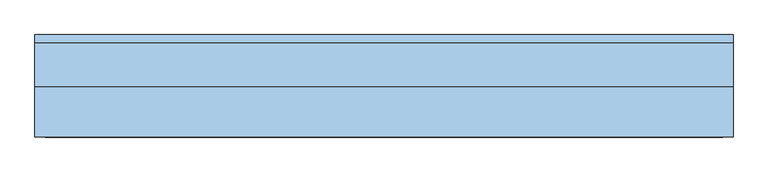
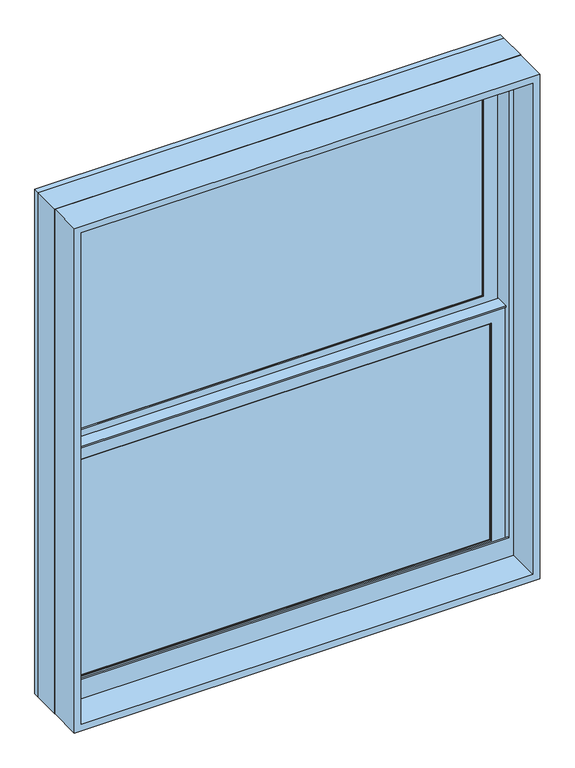
"""IFC4 building model written with IfcOpenShell, lengths in millimetres: window geometry, Window-Double_Hung-Marvin-Essential : ESDH3640."""

from ifc_helpers import new_model, si_unit, frame, origin, place, context, project, spatial, polyline, outline, extrude, faceted_brep, source, transform, mapped, element, save


def window_21e27111(model_context):
    return source(origin(), model_context, "Body", "SolidModel", [
        extrude(outline(polyline([(166.1583333, 20.6375), (166.1583333, 15.875), (147.1083333, 15.875), (147.1083333, 20.6375), (166.1583333, 20.6375)])), frame((0.0, 0.0, 1289.05), z_axis=(0.0, 0.0, 1.0), x_axis=(1.0, 0.0, 0.0)), (0.0, 0.0, 1.0), 527.05),
        extrude(outline(polyline([(-147.1083333, 20.6375), (-147.1083333, 15.875), (-166.1583333, 15.875), (-166.1583333, 20.6375), (-147.1083333, 20.6375)])), frame((0.0, 0.0, 1289.05), z_axis=(0.0, 0.0, 1.0), x_axis=(1.0, 0.0, 0.0)), (0.0, 0.0, 1.0), 527.05),
        extrude(outline(polyline([(469.9, 20.6375), (469.9, 15.875), (-469.9, 15.875), (-469.9, 20.6375), (469.9, 20.6375)])), frame((0.0, 0.0, 1543.05), z_axis=(0.0, 0.0, 1.0), x_axis=(1.0, 0.0, 0.0)), (0.0, 0.0, 1.0), 19.05),
        extrude(outline(polyline([(-166.1583333, 46.83125), (-166.1583333, 51.59375), (-147.1083333, 51.59375), (-147.1083333, 46.83125), (-166.1583333, 46.83125)])), frame((0.0, 0.0, 1854.2), z_axis=(0.0, 0.0, 1.0), x_axis=(1.0, 0.0, 0.0)), (0.0, 0.0, 1.0), 527.05),
        extrude(outline(polyline([(147.1083333, 46.83125), (147.1083333, 51.59375), (166.1583333, 51.59375), (166.1583333, 46.83125), (147.1083333, 46.83125)])), frame((0.0, 0.0, 1854.2), z_axis=(0.0, 0.0, 1.0), x_axis=(1.0, 0.0, 0.0)), (0.0, 0.0, 1.0), 527.05),
        extrude(outline(polyline([(-469.9, 46.83125), (-469.9, 51.59375), (469.9, 51.59375), (469.9, 46.83125), (-469.9, 46.83125)])), frame((0.0, 0.0, 2108.2), z_axis=(0.0, 0.0, 1.0), x_axis=(1.0, 0.0, 0.0)), (0.0, 0.0, 1.0), 19.05),
        extrude(outline(polyline([(166.1583333, 20.6375), (147.1083333, 20.6375), (147.1083333, 25.4), (166.1583333, 25.4), (166.1583333, 20.6375)])), frame((0.0, 0.0, 1289.05), z_axis=(0.0, 0.0, 1.0), x_axis=(1.0, 0.0, 0.0)), (0.0, 0.0, 1.0), 527.05),
        extrude(outline(polyline([(-147.1083333, 20.6375), (-166.1583333, 20.6375), (-166.1583333, 25.4), (-147.1083333, 25.4), (-147.1083333, 20.6375)])), frame((0.0, 0.0, 1289.05), z_axis=(0.0, 0.0, 1.0), x_axis=(1.0, 0.0, 0.0)), (0.0, 0.0, 1.0), 527.05),
        extrude(outline(polyline([(469.9, 20.6375), (-469.9, 20.6375), (-469.9, 25.4), (469.9, 25.4), (469.9, 20.6375)])), frame((0.0, 0.0, 1543.05), z_axis=(0.0, 0.0, 1.0), x_axis=(1.0, 0.0, 0.0)), (0.0, 0.0, 1.0), 19.05),
        extrude(outline(polyline([(-166.1583333, 56.35625), (-147.1083333, 56.35625), (-147.1083333, 51.59375), (-166.1583333, 51.59375), (-166.1583333, 56.35625)])), frame((0.0, 0.0, 1854.2), z_axis=(0.0, 0.0, 1.0), x_axis=(1.0, 0.0, 0.0)), (0.0, 0.0, 1.0), 527.05),
        extrude(outline(polyline([(147.1083333, 56.35625), (166.1583333, 56.35625), (166.1583333, 51.59375), (147.1083333, 51.59375), (147.1083333, 56.35625)])), frame((0.0, 0.0, 1854.2), z_axis=(0.0, 0.0, 1.0), x_axis=(1.0, 0.0, 0.0)), (0.0, 0.0, 1.0), 527.05),
        extrude(outline(polyline([(-469.9, 56.35625), (469.9, 56.35625), (469.9, 51.59375), (-469.9, 51.59375), (-469.9, 56.35625)])), frame((0.0, 0.0, 2108.2), z_axis=(0.0, 0.0, 1.0), x_axis=(1.0, 0.0, 0.0)), (0.0, 0.0, 1.0), 19.05),
        faceted_brep([(-496.8875, 5.6780605, 1846.1351748), (-496.8875, 5.6780605, 1841.5), (496.8875, 5.6780605, 1841.5), (496.8875, 5.6780605, 1846.1351748), (-496.8875, 34.8118605, 1846.1351748), (496.8875, 34.8118605, 1846.1351748), (496.8875, 34.8118605, 1841.5), (-496.8875, 34.8118605, 1841.5), (-496.8875, 30.1625, 1841.5), (-496.8875, 30.1625, 1262.0625), (-496.8875, 8.9241104, 1262.0625), (-496.8875, 8.9241104, 1841.5), (496.8875, 8.9241104, 1841.5), (496.8875, 30.1625, 1841.5), (496.8875, 8.9241104, 1262.0625), (496.8875, 30.1625, 1262.0625), (-481.0034752, 11.90625, 1827.2034752), (-481.0034752, 30.1625, 1827.2034752), (481.0034752, 30.1625, 1827.2034752), (481.0034752, 11.90625, 1827.2034752), (-464.34375, 10.4662439, 1810.54375), (-464.34375, 11.90625, 1810.54375), (464.34375, 11.90625, 1810.54375), (464.34375, 10.4662439, 1810.54375), (465.8858834, 8.9241104, 1812.0858834), (-465.8858834, 8.9241104, 1812.0858834), (481.0034752, 30.1625, 1277.9465248), (481.0034752, 11.90625, 1277.9465248), (464.34375, 11.90625, 1294.60625), (464.34375, 10.4662439, 1294.60625), (465.8858834, 8.9241104, 1293.0641166), (-481.0034752, 30.1625, 1277.9465248), (-481.0034752, 11.90625, 1277.9465248), (-464.34375, 11.90625, 1294.60625), (-464.34375, 10.4662439, 1294.60625), (-465.8858834, 8.9241104, 1293.0641166)], [[[0, 1, 2, 3]], [[4, 5, 6, 7]], [[1, 0, 4, 7, 8, 9, 10, 11]], [[2, 1, 11, 12]], [[7, 6, 13, 8]], [[3, 2, 12, 14, 15, 13, 6, 5]], [[0, 3, 5, 4]], [[16, 17, 18, 19]], [[20, 21, 22, 23]], [[20, 23, 24, 25]], [[19, 18, 26, 27]], [[23, 22, 28, 29]], [[24, 23, 29, 30]], [[27, 26, 31, 32]], [[29, 28, 33, 34]], [[30, 29, 34, 35]], [[15, 14, 10, 9]], [[15, 9, 8, 13], [18, 17, 31, 26]], [[17, 16, 32, 31]], [[16, 19, 27, 32], [22, 21, 33, 28]], [[21, 20, 34, 33]], [[20, 25, 35, 34]], [[10, 14, 12, 11], [25, 24, 30, 35]]]),
        extrude(outline(polyline([(38.5955581, 1827.2125), (33.5778968, 1827.2125), (33.5778968, 1828.8), (39.9405976, 1828.8), (39.9405976, 1827.2125), (61.515625, 1827.2125), (47.6307501, 1823.8975159), (38.5955581, 1823.8975159), (38.5955581, 1827.2125)])), frame((-496.8875, 0.0, 0.0), z_axis=(1.0, 0.0, 0.0), x_axis=(0.0, 1.0, 0.0)), (0.0, 0.0, 1.0), 993.775),
        faceted_brep([(527.05, 0.0, 1231.9), (527.05, 0.0, 2438.4), (-527.05, 0.0, 2438.4), (-527.05, 0.0, 1231.9), (500.85625, 0.0, 1293.01875), (-500.85625, 0.0, 1293.01875), (-500.85625, 0.0, 2412.20625), (500.85625, 0.0, 2412.20625), (500.85625, 3.96875, 1231.9), (-500.85625, 3.96875, 1231.9), (-500.85625, 3.96875, 1293.01875), (500.85625, 3.96875, 1293.01875), (-527.05, 65.6828125, 1231.9), (-500.85625, 65.6828125, 1231.9), (500.85625, 65.6828125, 1231.9), (527.05, 65.6828125, 1231.9), (-527.05, 65.6828125, 2438.4), (527.05, 65.6828125, 2438.4), (500.85625, 65.6828125, 2412.20625), (-500.85625, 65.6828125, 2412.20625)], [[[0, 1, 2, 3], [4, 5, 6, 7]], [[8, 9, 10, 11]], [[5, 4, 11, 10]], [[0, 3, 12, 13, 9, 8, 14, 15]], [[13, 12, 16, 17, 15, 14, 18, 19]], [[13, 19, 6, 5, 10, 9]], [[7, 6, 19, 18]], [[18, 14, 8, 11, 4, 7]], [[1, 0, 15, 17]], [[2, 1, 17, 16]], [[3, 2, 16, 12]]]),
        faceted_brep([(500.85625, 30.1625, 1835.15), (499.26875, 30.1625, 1835.15), (499.26875, 30.1625, 1256.2544613), (500.85625, 30.1625, 1256.2544613), (-499.26875, 30.1625, 1835.15), (-500.85625, 30.1625, 1835.15), (-500.85625, 30.1625, 1256.2544613), (-499.26875, 30.1625, 1256.2544613), (499.26875, 63.5, 1835.15), (500.85625, 63.5, 1835.15), (500.85625, 63.5, 1249.7743077), (499.26875, 63.5, 1249.7743077), (-500.85625, 63.5, 1835.15), (-499.26875, 63.5, 1835.15), (-499.26875, 63.5, 1249.7743077), (-500.85625, 63.5, 1249.7743077), (512.1108932, 3.96875, 1261.3460105), (512.1108932, 3.96875, 1231.9), (512.1108932, 65.6828125, 1231.9), (512.1108932, 65.6828125, 1249.350012), (-512.1108932, 3.96875, 1231.9), (-512.1108932, 3.96875, 1261.3460105), (-512.1108932, 65.6828125, 1249.350012), (-512.1108932, 65.6828125, 1231.9), (512.1108932, 78.58125, 1246.8428097), (-512.1108932, 78.58125, 1246.8428097), (-510.0971252, 68.2348864, 1248.8539391), (-492.13135, 68.2348864, 1248.8539391), (-492.13135, 65.6828125, 1249.350012), (492.13135, 65.6828125, 1249.350012), (492.13135, 68.2348864, 1248.8539391), (510.0971252, 68.2348864, 1248.8539391), (-527.05, 65.6828125, 1231.9), (-527.05, 78.5948249, 1231.9), (527.05, 78.5948249, 1231.9), (527.05, 65.6828125, 1231.9), (-527.05, 78.58125, 2438.4), (527.05, 78.58125, 2438.4), (512.1108932, 78.58125, 2423.4608932), (-512.1108932, 78.58125, 2423.4608932), (-527.05, 65.6828125, 2438.4), (-510.0971252, 68.2348864, 2421.4471252), (510.0971252, 68.2348864, 2421.4471252), (492.13135, 68.2348864, 2403.48135), (-492.13135, 68.2348864, 2403.48135), (-492.13135, 65.6828125, 2403.48135), (492.13135, 65.6828125, 2403.48135), (527.05, 65.6828125, 2438.4)], [[[0, 1, 2, 3]], [[4, 5, 6, 7]], [[8, 9, 10, 11]], [[12, 13, 14, 15]], [[1, 8, 11, 2]], [[9, 0, 3, 10]], [[1, 0, 9, 8]], [[5, 4, 13, 12]], [[5, 12, 15, 6]], [[13, 4, 7, 14]], [[16, 17, 18, 19]], [[20, 21, 22, 23]], [[24, 25, 26, 27, 28, 22, 21, 16, 19, 29, 30, 31], [3, 2, 11, 10], [7, 6, 15, 14]], [[17, 16, 21, 20]], [[17, 20, 23, 32, 33, 34, 35, 18]], [[34, 33, 36, 37], [25, 24, 38, 39]], [[33, 32, 40, 36]], [[39, 41, 26, 25]], [[41, 42, 31, 30, 43, 44, 27, 26]], [[44, 45, 28, 27]], [[40, 32, 23, 22, 28, 45, 46, 29, 19, 18, 35, 47]], [[36, 40, 47, 37]], [[39, 38, 42, 41]], [[44, 43, 46, 45]], [[34, 37, 47, 35]], [[42, 38, 24, 31]], [[46, 43, 30, 29]]]),
        extrude(outline(polyline([(477.04375, 11.90625), (-477.04375, 11.90625), (-477.04375, 15.08125), (477.04375, 15.08125), (477.04375, 11.90625)])), frame((0.0, 0.0, 1281.90625), z_axis=(0.0, 0.0, 1.0), x_axis=(1.0, 0.0, 0.0)), (0.0, 0.0, 1.0), 541.3375),
        extrude(outline(polyline([(477.04375, 42.8625), (-477.04375, 42.8625), (-477.04375, 46.0375), (477.04375, 46.0375), (477.04375, 42.8625)])), frame((0.0, 0.0, 1847.05625), z_axis=(0.0, 0.0, 1.0), x_axis=(1.0, 0.0, 0.0)), (0.0, 0.0, 1.0), 541.3375),
        faceted_brep([(-464.34375, 31.194477, 1810.54375), (-465.8858834, 32.7366104, 1812.0858834), (465.8858834, 32.7366104, 1812.0858834), (464.34375, 31.194477, 1810.54375), (-464.34375, 30.1625, 1810.54375), (464.34375, 30.1625, 1810.54375), (-496.8875, 32.7366104, 1843.0875), (-496.8875, 30.1625, 1843.0875), (496.8875, 30.1625, 1843.0875), (496.8875, 32.7366104, 1843.0875), (465.8858834, 32.7366104, 1293.0641166), (464.34375, 31.194477, 1294.60625), (464.34375, 30.1625, 1294.60625), (496.8875, 30.1625, 1262.0625), (496.8875, 32.7366104, 1262.0625), (-465.8858834, 32.7366104, 1293.0641166), (-464.34375, 31.194477, 1294.60625), (-464.34375, 30.1625, 1294.60625), (-496.8875, 30.1625, 1262.0625), (-496.8875, 32.7366104, 1262.0625)], [[[0, 1, 2, 3]], [[4, 0, 3, 5]], [[6, 7, 8, 9]], [[3, 2, 10, 11]], [[5, 3, 11, 12]], [[9, 8, 13, 14]], [[11, 10, 15, 16]], [[12, 11, 16, 17]], [[14, 13, 18, 19]], [[9, 14, 19, 6], [1, 15, 10, 2]], [[16, 15, 1, 0]], [[17, 16, 0, 4]], [[7, 18, 13, 8], [5, 12, 17, 4]], [[19, 18, 7, 6]]]),
        faceted_brep([(-481.0034752, 42.8625, 2392.3534752), (-481.0034752, 61.11875, 2392.3534752), (481.0034752, 61.11875, 2392.3534752), (481.0034752, 42.8625, 2392.3534752), (-464.34375, 41.4224939, 2375.69375), (-464.34375, 42.8625, 2375.69375), (464.34375, 42.8625, 2375.69375), (464.34375, 41.4224939, 2375.69375), (-465.8858834, 39.8803604, 2377.2358834), (465.8858834, 39.8803604, 2377.2358834), (-496.8875, 61.11875, 2408.2375), (-496.8875, 39.8803604, 2408.2375), (496.8875, 39.8803604, 2408.2375), (496.8875, 61.11875, 2408.2375), (481.0034752, 61.11875, 1843.0965248), (481.0034752, 42.8625, 1843.0965248), (464.34375, 42.8625, 1859.75625), (464.34375, 41.4224939, 1859.75625), (465.8858834, 39.8803604, 1858.2141166), (496.8875, 39.8803604, 1827.2125), (496.8875, 61.11875, 1827.2125), (-481.0034752, 61.11875, 1843.0965248), (-481.0034752, 42.8625, 1843.0965248), (-464.34375, 42.8625, 1859.75625), (-464.34375, 41.4224939, 1859.75625), (-465.8858834, 39.8803604, 1858.2141166), (-496.8875, 39.8803604, 1827.2125), (-496.8875, 61.11875, 1827.2125)], [[[0, 1, 2, 3]], [[4, 5, 6, 7]], [[8, 4, 7, 9]], [[10, 11, 12, 13]], [[3, 2, 14, 15]], [[7, 6, 16, 17]], [[9, 7, 17, 18]], [[13, 12, 19, 20]], [[15, 14, 21, 22]], [[17, 16, 23, 24]], [[18, 17, 24, 25]], [[20, 19, 26, 27]], [[13, 20, 27, 10], [1, 21, 14, 2]], [[22, 21, 1, 0]], [[3, 15, 22, 0], [5, 23, 16, 6]], [[24, 23, 5, 4]], [[25, 24, 4, 8]], [[11, 26, 19, 12], [9, 18, 25, 8]], [[27, 26, 11, 10]]]),
        faceted_brep([(-496.8875, 61.11875, 1827.2125), (-496.8875, 63.6928604, 1827.2125), (496.8875, 63.6928604, 1827.2125), (496.8875, 61.11875, 1827.2125), (-464.34375, 62.150727, 1859.75625), (-464.34375, 61.11875, 1859.75625), (464.34375, 61.11875, 1859.75625), (464.34375, 62.150727, 1859.75625), (-465.8858834, 63.6928604, 1858.2141166), (465.8858834, 63.6928604, 1858.2141166), (496.8875, 63.6928604, 2408.2375), (496.8875, 61.11875, 2408.2375), (464.34375, 61.11875, 2375.69375), (464.34375, 62.150727, 2375.69375), (465.8858834, 63.6928604, 2377.2358834), (-496.8875, 63.6928604, 2408.2375), (-496.8875, 61.11875, 2408.2375), (-464.34375, 61.11875, 2375.69375), (-464.34375, 62.150727, 2375.69375), (-465.8858834, 63.6928604, 2377.2358834)], [[[0, 1, 2, 3]], [[4, 5, 6, 7]], [[8, 4, 7, 9]], [[3, 2, 10, 11]], [[7, 6, 12, 13]], [[9, 7, 13, 14]], [[11, 10, 15, 16]], [[13, 12, 17, 18]], [[14, 13, 18, 19]], [[16, 15, 1, 0]], [[3, 11, 16, 0], [5, 17, 12, 6]], [[18, 17, 5, 4]], [[19, 18, 4, 8]], [[1, 15, 10, 2], [9, 14, 19, 8]]]),
        extrude(outline(polyline([(477.04375, 26.19375), (-477.04375, 26.19375), (-477.04375, 30.1625), (477.04375, 30.1625), (477.04375, 26.19375)])), frame((0.0, 0.0, 1281.90625), z_axis=(0.0, 0.0, 1.0), x_axis=(1.0, 0.0, 0.0)), (0.0, 0.0, 1.0), 541.3375),
        extrude(outline(polyline([(477.04375, 57.15), (-477.04375, 57.15), (-477.04375, 61.11875), (477.04375, 61.11875), (477.04375, 57.15)])), frame((0.0, 0.0, 1847.05625), z_axis=(0.0, 0.0, 1.0), x_axis=(1.0, 0.0, 0.0)), (0.0, 0.0, 1.0), 541.3375),
        extrude(outline(polyline([(2438.4, 527.05), (2438.4, -527.05), (1231.9, -527.05), (1231.9, 527.05), (2438.4, 527.05)]), holes=[polyline([(2422.525, 511.175), (1247.775, 511.175), (1247.775, -511.175), (2422.525, -511.175), (2422.525, 511.175)])]), frame((0.0, -76.2, 0.0), z_axis=(0.0, 1.0, 0.0), x_axis=(0.0, 0.0, 1.0)), (0.0, 0.0, 1.0), 75.40625),
    ])


if __name__ == "__main__":
    model = new_model("IFC4")
    model_context = context("Model", 3, world=origin())
    ifc_project = project(units=[si_unit("LENGTHUNIT", "METRE", prefix="MILLI")], contexts=[model_context])
    site = spatial("IfcSite", under=ifc_project)
    building = spatial("IfcBuilding", under=site)
    placement = place(None, origin())
    window_shape = window_21e27111(model_context)
    element("IfcWindow", 1, ObjectType="Window-Double_Hung-Marvin-Essential : ESDH3640", at=placement, inside=building, context=model_context, shape_type="MappedRepresentation", body=[
        mapped(window_shape, transform((0.0, 0.0, 0.0), x_axis=(1.0, 0.0, 0.0), y_axis=(0.0, 1.0, 0.0), z_axis=(0.0, 0.0, 1.0))),
    ])
    save(model, "model.ifc")

# Revit data of these elements
# Type "Window-Double_Hung-Marvin-Essential : ESDH3640"
#   Type Mark = "52"
#   Window Type = "Essential Double Hung"
#   Product data url = "https://bimobject.com/marvin-windows-and-doors/product/marvin-dhwau"
#   Product Guid = "c4a96547-874c-4385-91dc-a058adc19d98"
#   Frame = "All Ultrex"
#   Egress Window = "No"
#   URL = "www.marvin.com"
#   Model = "ESDH3640"
#   Manufacturer = "Marvin Windows and Doors"
#   Label Egress = ""
#   Glass Type = "IG Low E II with Argon"
#   Design Pressure = "DP50"
#   Description = "4248 DBHG"
#   Analytic Construction = "<None>"
#   Prairie Corner Width = 0' - 4"
#   Prairie Corner Height = 0' - 4"
#   Egress Width = 3' - 2 9/16"
#   Egress Height = 1' - 7 27/128"
#   Rough Width = 3' - 6"
#   Rough Height = 4' - 0"
#   Nominal Width = 3' - 6"
#   Nominal Height = 4' - 0"
#   Inset to Installation Flange [instance default] = 0' - 1"
#   Height = 3' - 11 1/2"
#   Egress Area = 5.1446 SF
#   Default Head Height = 8' - 0"
#   Width = 3' - 5 1/2"
#   Daylight Area = 10.3149 SF
#   DLO Width = 3' - 0 9/16"
#   DLO Height = 1' - 8 5/16"
#   Muntins Top Sash = yes
#   Lites Wide Top Sash = 3
#   Lites Wide Bottom Sash = 3
#   Lites High Top Sash = 2
#   Lites High Bottom Sash = 2
#   Lite Cut Prairie 9 = no
#   Lite Cut HV Grid = yes
#   Muntins Bottom Sash = yes
#   Label Visibility = no
#   Jamb Extension Visibility = yes
#   Edition number = 1
#   Interior Material = Ultrex-Marvin-Stonewhite
#   Glazing Material = Glass-Marvin-IG Low E II with Argon
#   Cladding Material = Ultrex-Marvin-Pebblegray
#   Wall Closure = (empty or 0)
#   Assembly Code = ""
# Element 1 (IfcWindow, "Window-Double_Hung-Marvin-Essential : ESDH3640")
#   Materials on its faces: "Ultrex-Marvin-Pebblegray", "Ultrex-Marvin-Stonewhite", "Glass-Marvin-IG Low E II with Argon"
# Materials
#   "Ultrex-Marvin-Stonewhite": class "Paint", colour RGB 250 251 245, transparency 0
#   "Glass-Marvin-IG Low E II with Argon": class "Glass", colour RGB 0 128 192, transparency 0.85
#   "Ultrex-Marvin-Pebblegray": class "Paint", colour RGB 189 185 173, transparency 0
